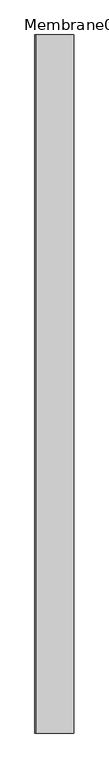
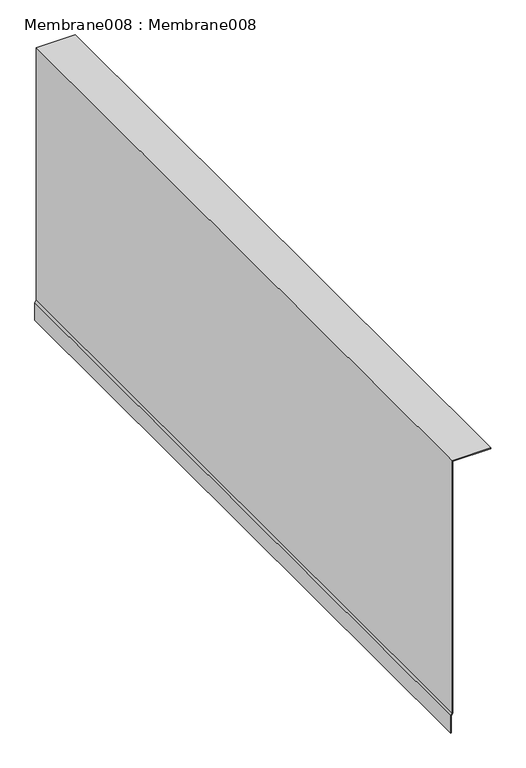
"""IFC4 building model written with IfcOpenShell, lengths in millimetres: proxy geometry, Membrane008 : Membrane008."""

from ifc_helpers import new_model, si_unit, frame, origin, place, context, project, spatial, polyline, outline, extrude, source, transform, mapped, element, save


def membrane008_membrane008_11970a71(model_context):
    return source(origin(), model_context, "Body", "SweptSolid", [
        extrude(outline(polyline([(33543.7417519, -9680.9523707), (33550.7495644, -9676.7926596), (34290.438014, -9676.7926596), (34290.438014, -9570.993191), (34291.938014, -9570.993191), (34291.938014, -9678.2926596), (33551.1612212, -9678.2926596), (33544.1534087, -9682.4523707), (33493.9487832, -9682.4523707), (33493.9487832, -9680.9523707), (33543.7417519, -9680.9523707)])), frame((0.0, 7182.1529359, 0.0), z_axis=(0.0, 1.0, 0.0), x_axis=(0.0, 0.0, 1.0)), (0.0, 0.0, 1.0), 2000.0),
    ])


if __name__ == "__main__":
    model = new_model("IFC4")
    model_context = context("Model", 3, world=origin())
    ifc_project = project(units=[si_unit("LENGTHUNIT", "METRE", prefix="MILLI")], contexts=[model_context])
    site = spatial("IfcSite", under=ifc_project)
    building = spatial("IfcBuilding", under=site)
    placement = place(None, origin())
    membrane008_membrane008_shape = membrane008_membrane008_11970a71(model_context)
    element("IfcBuildingElementProxy", 1, Name="Membrane008 : Membrane008", ObjectType="Membrane008 : Membrane008", at=placement, inside=building, context=model_context, shape_type="MappedRepresentation", body=[
        mapped(membrane008_membrane008_shape, transform((0.0, 0.0, 0.0), x_axis=(1.0, 0.0, 0.0), y_axis=(0.0, 1.0, 0.0), z_axis=(0.0, 0.0, 1.0))),
    ])
    save(model, "model.ifc")

# Revit data of these elements
# Type "Membrane008 : Membrane008"
#   NameOverride = "Membrane008"
# Element 1 (IfcBuildingElementProxy, "Membrane008 : Membrane008")
#   Materials on its faces: "(2) LAYERS OF ICE & WATER SHIELD (BITUTHANE) UNDER STUCCO"
# Materials
#   "(2) LAYERS OF ICE & WATER SHIELD (BITUTHANE) UNDER STUCCO": class "Unassigned", colour RGB 186 255 159, transparency 0, Cost = 0
